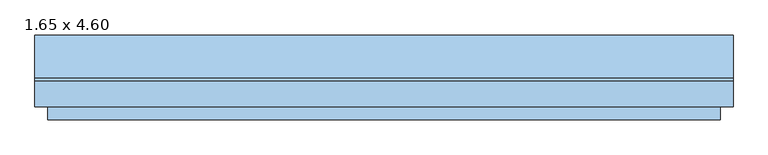
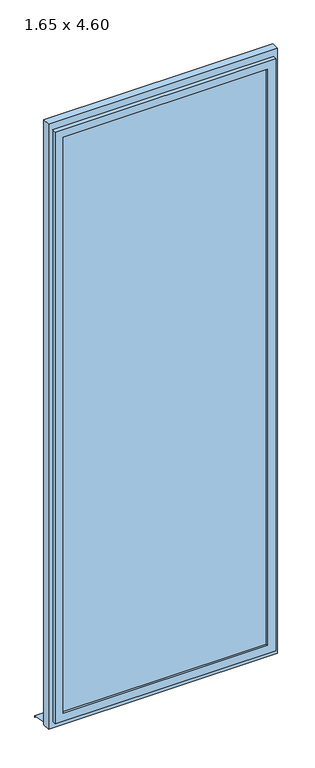
"""IFC4 building model written with IfcOpenShell, lengths in millimetres: window geometry, Fenstertür 1-flg : 1.65 x 4.60."""

from ifc_helpers import new_model, si_unit, frame, origin, place, context, project, spatial, polyline, outline, extrude, faceted_brep, source, transform, mapped, element, save


def window_1_65_x_4_60_d3fc4a1d(model_context):
    return source(origin(), model_context, "Body", "SolidModel", [
        extrude(outline(polyline([(4600.0, 825.0), (4600.0, -825.0), (0.0, -825.0), (0.0, 825.0), (4600.0, 825.0)]), holes=[polyline([(4520.0, 765.0), (80.0, 765.0), (80.0, -765.0), (4520.0, -765.0), (4520.0, 765.0)])]), frame((0.0, -80.0, 0.0), z_axis=(0.0, 1.0, 0.0), x_axis=(0.0, 0.0, 1.0)), (0.0, 0.0, 1.0), 60.0),
        faceted_brep([(795.0, -80.0, 4550.0), (795.0, -110.0, 4550.0), (795.0, -110.0, 50.0), (795.0, -80.0, 50.0), (-795.0, -110.0, 4550.0), (-795.0, -110.0, 50.0), (735.0, -110.0, 110.0), (-735.0, -110.0, 110.0), (-735.0, -110.0, 4490.0), (735.0, -110.0, 4490.0), (-795.0, -80.0, 50.0), (-795.0, -80.0, 4550.0), (765.0, -80.0, 4520.0), (-765.0, -80.0, 4520.0), (-765.0, -80.0, 80.0), (765.0, -80.0, 80.0), (765.0, -50.0, 4520.0), (765.0, -50.0, 80.0), (-765.0, -50.0, 80.0), (-765.0, -50.0, 4520.0), (735.0, -50.0, 4490.0), (-735.0, -50.0, 4490.0), (-735.0, -50.0, 110.0), (735.0, -50.0, 110.0)], [[[0, 1, 2, 3]], [[1, 4, 5, 2], [6, 7, 8, 9]], [[3, 2, 5, 10]], [[3, 10, 11, 0], [12, 13, 14, 15]], [[16, 12, 15, 17]], [[17, 15, 14, 18]], [[17, 18, 19, 16], [20, 21, 22, 23]], [[9, 20, 23, 6]], [[6, 23, 22, 7]], [[10, 5, 4, 11]], [[18, 14, 13, 19]], [[7, 22, 21, 8]], [[11, 4, 1, 0]], [[19, 13, 12, 16]], [[8, 21, 20, 9]]]),
        extrude(outline(polyline([(-9.9778457, 20.0), (90.0, 0.0), (90.0, -10.0), (88.0, -10.0), (88.0, -1.6395366), (-10.1759277, 18.0), (-20.0, 18.0), (-20.0, 20.0), (-9.9778457, 20.0)])), frame((-825.0, 0.0, 0.0), z_axis=(1.0, 0.0, 0.0), x_axis=(0.0, 1.0, 0.0)), (0.0, 0.0, 1.0), 1650.0),
        extrude(outline(polyline([(735.0, -95.0), (-735.0, -95.0), (-735.0, -65.0), (735.0, -65.0), (735.0, -95.0)])), frame((0.0, 0.0, 110.0), z_axis=(0.0, 0.0, 1.0), x_axis=(1.0, 0.0, 0.0)), (0.0, 0.0, 1.0), 4380.0),
    ])


if __name__ == "__main__":
    model = new_model("IFC4")
    model_context = context("Model", 3, world=origin())
    ifc_project = project(units=[si_unit("LENGTHUNIT", "METRE", prefix="MILLI")], contexts=[model_context])
    site = spatial("IfcSite", under=ifc_project)
    building = spatial("IfcBuilding", under=site)
    placement = place(None, origin())
    window_1_65_x_4_60_shape = window_1_65_x_4_60_d3fc4a1d(model_context)
    element("IfcWindow", 1, ObjectType="Fenstertür 1-flg : 1.65 x 4.60", at=placement, inside=building, context=model_context, shape_type="MappedRepresentation", body=[
        mapped(window_1_65_x_4_60_shape, transform((0.0, 0.0, 0.0), x_axis=(1.0, 0.0, 0.0), y_axis=(0.0, 1.0, 0.0), z_axis=(0.0, 0.0, 1.0))),
    ])
    save(model, "model.ifc")

# Revit data of these elements
# Type "Fenstertür 1-flg : 1.65 x 4.60"
#   Type Mark = "57"
#   Operation = "SinglePanel"
#   Construction Type Id = "SGL"
#   Keynote = "16.05.01"
#   Analytic Construction = "Große Fenster mit Einfachverglasung"
#   Visual Light Transmittance = 0.9
#   Solar Heat Gain Coefficient = 0.86
#   Rough Width = 1.650 m
#   Rough Height = 4.600 m
#   Heat Transfer Coefficient (U) = 5.5617 W/(m²·K)
#   Rahmentiefe = 0.060 m
#   Rahmenhöhe unten = 0.080 m
#   Höhe oberer  Rahmen = 0.080 m
#   Rahmenbreite = 0.060 m
#   Height = 4.600 m
#   Tiefe Flügel = 0.060 m
#   Flügelbreite = 0.060 m
#   Einbautiefe (von außen) [instance default] = 0.080 m
#   Width = 1.650 m
#   Sichtbarkeit Sturzlinien [instance default] = yes
#   Öffnungsrichtung oben [instance default] = yes
#   Öffnungsrichtung in Draufsicht anzeigen [instance default] = yes
#   Drehflügel 1 [instance default] = yes
#   Bild [instance default] = none
#   Glas [instance default] = none
#   Fensterflügel [instance default] = none
#   Äußere Fensterbank [instance default] = none
#   Wall Closure = (empty or 0)
# Element 1 (IfcWindow, "Fenstertür 1-flg : 1.65 x 4.60")
#   Materials on its faces: "Kunststoff - Weiß", "Glas"
# Materials
#   "Kunststoff - Weiß": class "Kunststoff", colour RGB 249 249 249, transparency 0, Cost = 0
#   "Glas": class "Glas", colour RGB 0 0 255, transparency 0.75, Comments = "Render-Darstellung nicht aktualisiert ", Cost = 0
